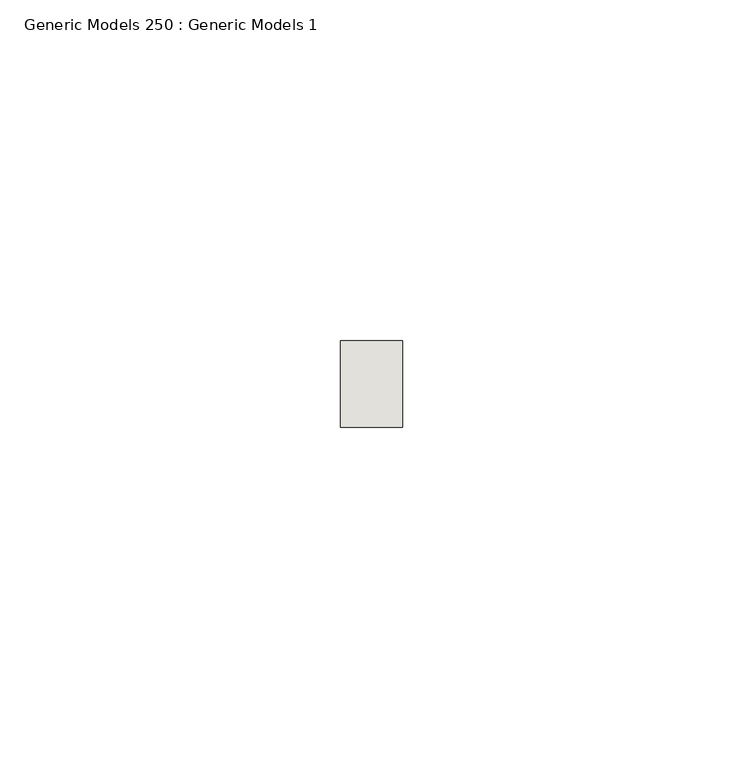
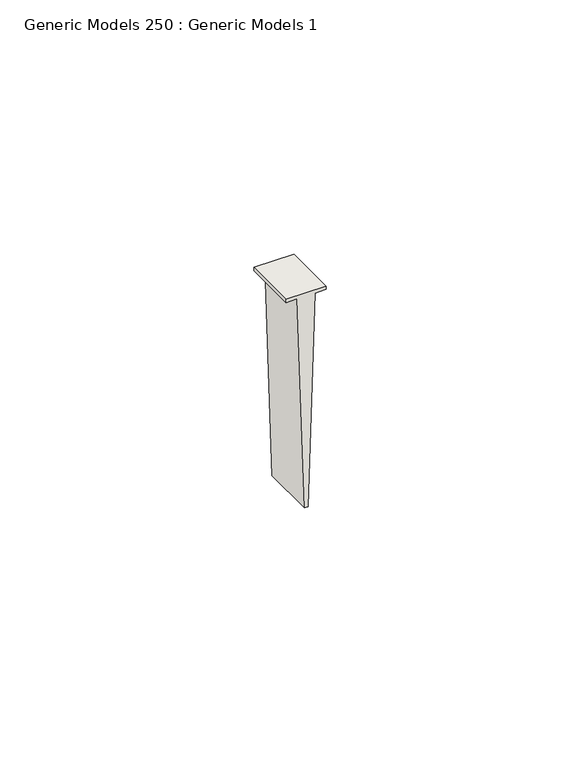
"""IFC4 building model written with IfcOpenShell, lengths in millimetres: wall geometry, Generic Models 250 : Generic Models 1."""

from ifc_helpers import new_model, si_unit, frame, origin, place, context, project, spatial, polyline, outline, extrude, source, transform, mapped, element, save


def generic_models_250_generic_models_1_0176a329(model_context):
    return source(origin(), model_context, "Body", "SweptSolid", [
        extrude(outline(polyline([(3050.38125, 49733.4159), (3049.5875, 49733.4159), (3049.5875, 49735.9657636), (2998.7875, 49737.5631527), (2998.7875, 49738.3618473), (3049.5875, 49739.9592364), (3049.5875, 49742.5091), (3050.38125, 49742.5091), (3050.38125, 49733.4159)])), frame((0.0, 565.15, 0.0), z_axis=(0.0, 1.0, 0.0), x_axis=(0.0, 0.0, 1.0)), (0.0, 0.0, 1.0), 12.7),
    ])


if __name__ == "__main__":
    model = new_model("IFC4")
    model_context = context("Model", 3, world=origin())
    ifc_project = project(units=[si_unit("LENGTHUNIT", "METRE", prefix="MILLI")], contexts=[model_context])
    site = spatial("IfcSite", under=ifc_project)
    building = spatial("IfcBuilding", under=site)
    placement = place(None, origin())
    generic_models_250_generic_models_1_shape = generic_models_250_generic_models_1_0176a329(model_context)
    element("IfcWall", 1, ObjectType="Generic Models 250 : Generic Models 1", at=placement, inside=building, context=model_context, shape_type="MappedRepresentation", body=[
        mapped(generic_models_250_generic_models_1_shape, transform((0.0, 0.0, 0.0), x_axis=(1.0, 0.0, 0.0), y_axis=(0.0, 1.0, 0.0), z_axis=(0.0, 0.0, 1.0))),
    ])
    save(model, "model.ifc")

# Revit data of these elements
# Element 1 (IfcWall, "Generic Models 250 : Generic Models 1")
#   Materials on its faces: "METAL RUNNER CHANNEL; FASTEN @ 24\" O.C."
# Materials
#   "METAL RUNNER CHANNEL; FASTEN @ 24\" O.C.": class "Unassigned", colour RGB 210 209 208, transparency 0, Keynote = "M05121300.02", Cost = 0
